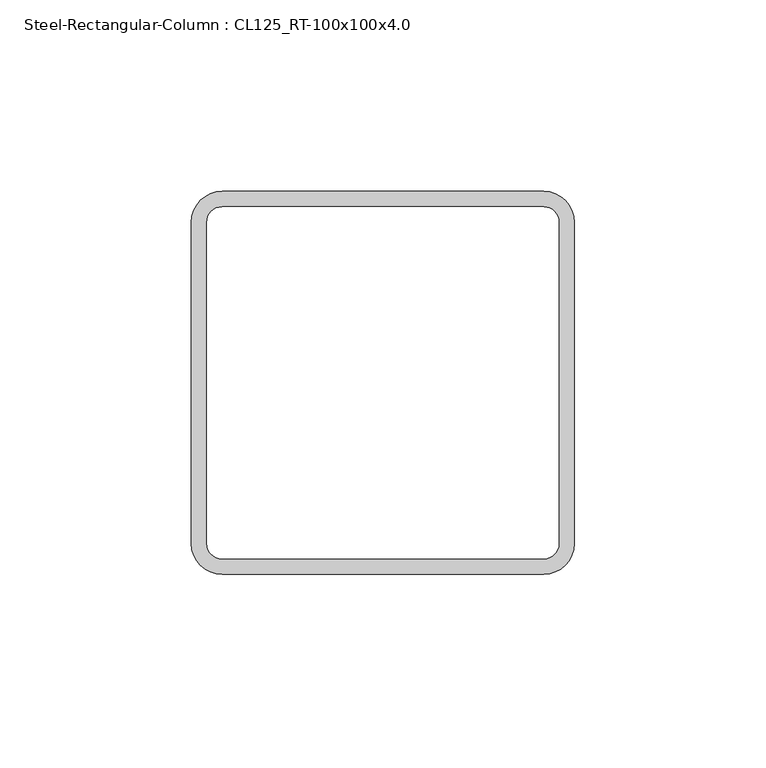
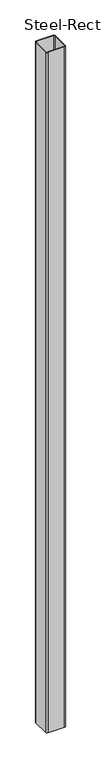
"""IFC4 building model written with IfcOpenShell, lengths in millimetres: column geometry, Steel-Rectangular-Column : CL125_RT-100x100x4.0."""

import ifcopenshell
import ifcopenshell.guid

model = None  # the IFC model being written
_history = None  # IfcOwnerHistory: only IFC2X3 demands one
_inside = {}  # id of a spatial element -> (the spatial element, [elements in it])
_under = {}  # id of a project, library or spatial element -> (it, [spatial elements below it])
_declared = {}  # id of a project -> (the project, [libraries it declares])
_typed = {}  # id of a type object -> (the type object, [elements of that type])
_made_of = {}  # id of a material, layer set ... -> (it, [elements and type objects made of it])


def new_model(schema):
    """Start an empty IFC model of exactly this schema.

    Asked for "IFC4X3", IfcOpenShell would pick the latest addendum, in which some entities
    have other attributes; the version numbers below select the first issue.
    IFC2X3 requires an IfcOwnerHistory on every rooted entity: one is made here for all.
    """
    global model, _history
    if schema == "IFC4X3":
        model = ifcopenshell.file(schema_version=(4, 3, 0, 0))
    else:
        model = ifcopenshell.file(schema=schema)
    _inside.clear()
    _under.clear()
    _declared.clear()
    _typed.clear()
    _made_of.clear()
    _history = None
    if model.schema == "IFC2X3":
        org = make("IfcOrganization", Name="unknown")
        user = make(
            "IfcPersonAndOrganization",
            ThePerson=make("IfcPerson", FamilyName="unknown"),
            TheOrganization=org,
        )
        app = make(
            "IfcApplication",
            ApplicationDeveloper=org,
            Version="unknown",
            ApplicationFullName="unknown",
            ApplicationIdentifier="unknown",
        )
        _history = make(
            "IfcOwnerHistory",
            OwningUser=user,
            OwningApplication=app,
            ChangeAction="ADDED",
            CreationDate=0,
        )
    return model


def make(cls, **values):
    """One entity of the class cls with the attributes given. An attribute that is None is left unset."""
    return model.create_entity(
        cls, **{name: value for name, value in values.items() if value is not None}
    )


def rooted(cls, **values):
    """An entity with a GlobalId (a new one), such as an element, a storey or a relation."""
    return make(cls, GlobalId=ifcopenshell.guid.new(), OwnerHistory=_history, **values)


def si_unit(unit_type, name, prefix=None):
    """IfcSIUnit, for example si_unit("LENGTHUNIT", "METRE", prefix="MILLI")."""
    return make("IfcSIUnit", UnitType=unit_type, Prefix=prefix, Name=name)


def assignment(units):
    """IfcUnitAssignment: the units of a project."""
    return None if units is None else make("IfcUnitAssignment", Units=units)


def point(xyz):
    """IfcCartesianPoint."""
    return None if xyz is None else make("IfcCartesianPoint", Coordinates=xyz)


def direction(xyz):
    """IfcDirection."""
    return None if xyz is None else make("IfcDirection", DirectionRatios=xyz)


def frame(location, z_axis=None, x_axis=None):
    """IfcAxis2Placement3D, a coordinate frame: its origin and axes. An axis left out is left unset."""
    return make(
        "IfcAxis2Placement3D",
        Location=point(location),
        Axis=direction(z_axis),
        RefDirection=direction(x_axis),
    )


def frame_2d(location, x_axis=None):
    """IfcAxis2Placement2D, a coordinate frame in the plane: its origin and x axis."""
    return make(
        "IfcAxis2Placement2D", Location=point(location), RefDirection=direction(x_axis)
    )


def origin():
    """The frame at (0, 0, 0) with its axes left unset."""
    return frame((0.0, 0.0, 0.0))


def place(relative_to, where):
    """IfcLocalPlacement: puts the frame where relative to a parent placement (None: the world)."""
    return make(
        "IfcLocalPlacement", PlacementRelTo=relative_to, RelativePlacement=where
    )


def context(
    kind, dimensions, precision=None, world=None, true_north=None, identifier=None
):
    """IfcGeometricRepresentationContext, for example the 3D "Model" context."""
    return make(
        "IfcGeometricRepresentationContext",
        ContextIdentifier=identifier,
        ContextType=kind,
        CoordinateSpaceDimension=dimensions,
        Precision=precision,
        WorldCoordinateSystem=world,
        TrueNorth=true_north,
    )


def project(units=None, contexts=None):
    """IfcProject with its units and contexts."""
    return rooted(
        "IfcProject",
        Name="project",
        RepresentationContexts=contexts,
        UnitsInContext=assignment(units),
    )


def spatial(cls, under=None, at=None, **own):
    """A site, building, storey or space (cls), placed at a placement, below another one or the project."""
    s = rooted(cls, ObjectPlacement=at, **own)
    if under is not None:
        _under.setdefault(under.id(), (under, []))[1].append(s)
    return s


def polyline(points):
    """IfcPolyline through the points."""
    return make("IfcPolyline", Points=[point(p) for p in points])


def circle_curve(where, radius):
    """IfcCircle in the frame where."""
    return make("IfcCircle", Position=where, Radius=radius)


def trimmed(basis, trim1, trim2, sense, master):
    """IfcTrimmedCurve: the piece of a basis curve between two trims."""
    return make(
        "IfcTrimmedCurve",
        BasisCurve=basis,
        Trim1=trim1,
        Trim2=trim2,
        SenseAgreement=sense,
        MasterRepresentation=master,
    )


def segment(curve, same_sense, transition):
    """IfcCompositeCurveSegment."""
    return make(
        "IfcCompositeCurveSegment",
        Transition=transition,
        SameSense=same_sense,
        ParentCurve=curve,
    )


def composite_curve(segments, self_intersect=None):
    """IfcCompositeCurve: segments joined end to end."""
    return make("IfcCompositeCurve", Segments=segments, SelfIntersect=self_intersect)


def outline(outer, holes=None, kind="AREA"):
    """IfcArbitraryClosedProfileDef: a profile drawn as a closed curve; with holes, ...WithVoids."""
    if holes is None:
        return make("IfcArbitraryClosedProfileDef", ProfileType=kind, OuterCurve=outer)
    return make(
        "IfcArbitraryProfileDefWithVoids",
        ProfileType=kind,
        OuterCurve=outer,
        InnerCurves=holes,
    )


def extrude(swept, where, along, depth):
    """IfcExtrudedAreaSolid: the profile swept, set in the frame where, extruded along a direction by depth."""
    return make(
        "IfcExtrudedAreaSolid",
        SweptArea=swept,
        Position=where,
        ExtrudedDirection=direction(along),
        Depth=depth,
    )


def shape(context_of_items, identifier, shape_type, items):
    """IfcShapeRepresentation: the items that make up one representation, for example the "Body"."""
    return make(
        "IfcShapeRepresentation",
        ContextOfItems=context_of_items,
        RepresentationIdentifier=identifier,
        RepresentationType=shape_type,
        Items=items,
    )


def source(mapping_origin, context_of_items, identifier, shape_type, items):
    """IfcRepresentationMap: a shape defined once, which mapped items show again and again."""
    return make(
        "IfcRepresentationMap",
        MappingOrigin=mapping_origin,
        MappedRepresentation=shape(context_of_items, identifier, shape_type, items),
    )


def transform(
    local_origin,
    x_axis=None,
    y_axis=None,
    z_axis=None,
    scale=None,
    scale2=None,
    scale3=None,
    uniform=True,
):
    """IfcCartesianTransformationOperator3D, or its non-uniform kind. x_axis, y_axis, z_axis: its Axis1, 2, 3."""
    if uniform:
        return make(
            "IfcCartesianTransformationOperator3D",
            Axis1=direction(x_axis),
            Axis2=direction(y_axis),
            LocalOrigin=point(local_origin),
            Scale=scale,
            Axis3=direction(z_axis),
        )
    return make(
        "IfcCartesianTransformationOperator3DnonUniform",
        Axis1=direction(x_axis),
        Axis2=direction(y_axis),
        LocalOrigin=point(local_origin),
        Scale=scale,
        Axis3=direction(z_axis),
        Scale2=scale2,
        Scale3=scale3,
    )


def mapped(mapping_source, mapping_target):
    """IfcMappedItem: shows the shape of a source again, moved by a transform."""
    return make(
        "IfcMappedItem", MappingSource=mapping_source, MappingTarget=mapping_target
    )


def made_of(thing, what):
    """Note that an element or type object is made of a material, layer set ...; save() writes the relation."""
    if what is not None:
        _made_of.setdefault(what.id(), (what, []))[1].append(thing)
    return thing


def element(
    cls,
    number,
    at=None,
    inside=None,
    cuts=None,
    type_object=None,
    material=None,
    context=None,
    identifier="Body",
    shape_type=None,
    held_by="IfcProductDefinitionShape",
    body=None,
    shapes=None,
    **own,
):
    """One element of the class cls, such as IfcWall. Its Tag is "e" and its number.

    at: its placement. inside: the storey or other place that contains it. cuts: it is an
    opening in that element (IfcRelVoidsElement). A single representation is given by context,
    identifier, shape_type and body (its items); several are given by shapes. held_by: the class
    of the entity that holds the representations. save() writes the other relations.
    """
    e = rooted(cls, Tag="e%d" % number, ObjectPlacement=at, **own)
    if body is not None:
        shapes = [shape(context, identifier, shape_type, body)]
    if shapes is not None:
        e.Representation = make(held_by, Representations=shapes)
    if inside is not None:
        _inside.setdefault(inside.id(), (inside, []))[1].append(e)
    if cuts is not None:
        rooted(
            "IfcRelVoidsElement", RelatingBuildingElement=cuts, RelatedOpeningElement=e
        )
    if type_object is not None:
        _typed.setdefault(type_object.id(), (type_object, []))[1].append(e)
    return made_of(e, material)


def aggregate(whole, parts):
    """IfcRelAggregates: a whole, such as a stair, and the parts it consists of."""
    return rooted("IfcRelAggregates", RelatingObject=whole, RelatedObjects=parts)


def save(model, path):
    """Write the relations noted so far, then the file.

    IfcRelAggregates (storeys below a building ...), IfcRelContainedInSpatialStructure (elements
    in a storey), IfcRelDefinesByType, IfcRelAssociatesMaterial and IfcRelDeclares: one each for
    every whole, place, type object, material and project.
    """
    for whole, parts in _under.values():
        aggregate(whole, parts)
    for where, things in _inside.values():
        rooted(
            "IfcRelContainedInSpatialStructure",
            RelatedElements=things,
            RelatingStructure=where,
        )
    for kind, things in _typed.values():
        rooted("IfcRelDefinesByType", RelatedObjects=things, RelatingType=kind)
    for what, things in _made_of.values():
        rooted("IfcRelAssociatesMaterial", RelatedObjects=things, RelatingMaterial=what)
    for by, libraries in _declared.values():
        rooted("IfcRelDeclares", RelatingContext=by, RelatedDefinitions=libraries)
    model.write(path)


def steel_rectangular_column_cl125_rt_100x100x4_0_3623087c(model_context):
    return source(origin(), model_context, "Body", "SweptSolid", [
        extrude(outline(composite_curve([segment(polyline([(42.0, -50.0), (-42.0, -50.0)]), True, "CONTINUOUS"), segment(trimmed(circle_curve(frame_2d((-42.0, -42.0)), 8.0), [point((-42.0, -50.0))], [point((-50.0, -42.0))], False, "CARTESIAN"), True, "CONTINUOUS"), segment(polyline([(-50.0, -42.0), (-50.0, 42.0)]), True, "CONTINUOUS"), segment(trimmed(circle_curve(frame_2d((-42.0, 42.0)), 8.0), [point((-50.0, 42.0))], [point((-42.0, 50.0))], False, "CARTESIAN"), True, "CONTINUOUS"), segment(polyline([(-42.0, 50.0), (42.0, 50.0)]), True, "CONTINUOUS"), segment(trimmed(circle_curve(frame_2d((42.0, 42.0)), 8.0), [point((42.0, 50.0))], [point((50.0, 42.0))], False, "CARTESIAN"), True, "CONTINUOUS"), segment(polyline([(50.0, 42.0), (50.0, -42.0)]), True, "CONTINUOUS"), segment(trimmed(circle_curve(frame_2d((42.0, -42.0)), 8.0), [point((50.0, -42.0))], [point((42.0, -50.0))], False, "CARTESIAN"), True, "CONTINUOUS")], self_intersect=False), holes=[composite_curve([segment(trimmed(circle_curve(frame_2d((42.0, -42.0)), 4.0), [point((42.0, -46.0))], [point((46.0, -42.0))], True, "CARTESIAN"), True, "CONTINUOUS"), segment(polyline([(46.0, -42.0), (46.0, 42.0)]), True, "CONTINUOUS"), segment(trimmed(circle_curve(frame_2d((42.0, 42.0)), 4.0), [point((46.0, 42.0))], [point((42.0, 46.0))], True, "CARTESIAN"), True, "CONTINUOUS"), segment(polyline([(42.0, 46.0), (-42.0, 46.0)]), True, "CONTINUOUS"), segment(trimmed(circle_curve(frame_2d((-42.0, 42.0)), 4.0), [point((-42.0, 46.0))], [point((-46.0, 42.0))], True, "CARTESIAN"), True, "CONTINUOUS"), segment(polyline([(-46.0, 42.0), (-46.0, -42.0)]), True, "CONTINUOUS"), segment(trimmed(circle_curve(frame_2d((-42.0, -42.0)), 4.0), [point((-46.0, -42.0))], [point((-42.0, -46.0))], True, "CARTESIAN"), True, "CONTINUOUS"), segment(polyline([(-42.0, -46.0), (42.0, -46.0)]), True, "CONTINUOUS")], self_intersect=False)]), frame((0.0, 0.0, 1400.0), z_axis=(0.0, 0.0, 1.0), x_axis=(1.0, 0.0, 0.0)), (0.0, 0.0, 1.0), 3600.0),
    ])


if __name__ == "__main__":
    model = new_model("IFC4")
    model_context = context("Model", 3, world=origin())
    ifc_project = project(units=[si_unit("LENGTHUNIT", "METRE", prefix="MILLI")], contexts=[model_context])
    site = spatial("IfcSite", under=ifc_project)
    building = spatial("IfcBuilding", under=site)
    placement = place(None, origin())
    steel_rectangular_column_cl125_rt_100x100x4_0_shape = steel_rectangular_column_cl125_rt_100x100x4_0_3623087c(model_context)
    element("IfcColumn", 1, ObjectType="Steel-Rectangular-Column : CL125_RT-100x100x4.0", at=placement, inside=building, context=model_context, shape_type="MappedRepresentation", body=[
        mapped(steel_rectangular_column_cl125_rt_100x100x4_0_shape, transform((0.0, 0.0, 0.0), x_axis=(1.0, 0.0, 0.0), y_axis=(0.0, 1.0, 0.0), z_axis=(0.0, 0.0, 1.0))),
    ])
    save(model, "model.ifc")

# Revit data of these elements
# Project information
#   Project ISM Data = "<?xml version=\"1.0\" encoding=\"utf-16\"?><ism schema_version=\"03.00\"><section_positioning><element family_name=\"CO_RC_REC\" symbol_name=\"CCC12_Rec_450x450\" section_id=\"F2ADF140-E21A-4820-8170-6F63D956DCAD\" category=\"OST_StructuralColumns\" mirror_y=\"0\" mirror_x=\"0\" /><element family_name=\"CO_RC_REC\" symbol_name=\"CCC12_Rec_450x450\" section_id=\"B35A310E-4F33-462b-819C-3ADD300C0CEB\" category=\"OST_StructuralColumns\" mirror_y=\"0\" mirror_x=\"0\" /><element family_name=\"CO_RC_REC\" symbol_name=\"CCC12_Rec_450x450\" section_id=\"711054EC-0DB2-46e3-AD20-004560300C00\" category=\"OST_StructuralColumns\" mirror_y=\"0\" mirror_x=\"0\" /><element family_name=\"CO_RC_REC\" symbol_name=\"300 x 450\" section_id=\"B5C54EC9-8EBD-4860-AB72-EF5791AED394\" category=\"OST_StructuralColumns\" mirror_y=\"0\" mirror_x=\"0\" /><element family_name=\"GI_RC_C\" symbol_name=\"SGC11_400x500\" section_id=\"0A7B8D02-9EA4-4aa9-A41A-E30BB5B6B6C5\" category=\"OST_StructuralFraming\" mirror_y=\"0\" mirror_x=\"0\" /><element family_name=\"GI_RC_C\" symbol_name=\"SGC11_400x500\" section_id=\"714BBD27-DB58-47da-B54C-5806291C2D3C\" category=\"OST_StructuralFraming\" mirror_y=\"0\" mirror_x=\"0\" /><element family_name=\"GI_RC_C\" symbol_name=\"SGC11_400x500\" section_id=\"F36E62C1-13EE-4807-A3C1-899E23E0BEDE\" category=\"OST_StructuralFraming\" mirror_y=\"0\" mirror_x=\"0\" /><element family_name=\"GI_RC_C\" symbol_name=\"SGC11_400x500\" section_id=\"F5448801-679E-44d6-8F46-E676344F8165\" category=\"OST_StructuralFraming\" mirror_y=\"0\" mirror_x=\"0\" /><element family_name=\"GI_RC_C\" symbol_name=\"SGC11_400x600\" section_id=\"05D74241-6318-4cac-95F5-7B878260D5B5\" category=\"OST_StructuralFraming\" mirror_y=\"0\" mirror_x=\"0\" /><element family_name=\"GI_RC_C\" symbol_name=\"SGC11_400x500\" section_id=\"846DCB0C-E06B-4978-9D43-E1CC0FDE7595\" category=\"OST_StructuralFraming\" mirror_y=\"0\" mirror_x=\"0\" /><element family_name=\"GI_RC_C\" symbol_name=\"SGC11_400x500\" section_id=\"2ADF82B8-986D-4f44-85DE-89D921292160\" category=\"OST_StructuralFraming\" mirror_y=\"0\" mirror_x=\"0\" /><element family_name=\"GI_RC_C\" symbol_name=\"SGC11_400x500\" section_id=\"7AF371ED-051B-4a30-8826-11F11C212B73\" category=\"OST_StructuralFraming\" mirror_y=\"0\" mirror_x=\"0\" /><element family_name=\"GI_RC_C\" symbol_name=\"SGC11_400x500\" section_id=\"2FE74006-ADDA-412f-A522-853919E62B4D\" category=\"OST_StructuralFraming\" mirror_y=\"0\" mirror_x=\"0\" /><element family_name=\"GI_RC_C\" symbol_name=\"SGC11_400x500\" section_id=\"09B63641-D581-4a6c-A18E-54C17EC989A4\" category=\"OST_StructuralFraming\" mirror_y=\"0\" mirror_x=\"0\" /><element family_name=\"GI_RC_C\" symbol_name=\"SGC11_400x500\" section_id=\"0DD6B52A-77D0-45a1-82B1-8236ED57078C\" category=\"OST_StructuralFraming\" mirror_y=\"0\" mirror_x=\"0\" /><element family_name=\"GI_RC_C\" symbol_name=\"SGC11_400x500\" section_id=\"35D311D2-DEB8-4469-97DE-110B6DF5B84D\" category=\"OST_StructuralFraming\" mirror_y=\"0\" mirror_x=\"0\" /><element family_name=\"GI_RC_C\" symbol_name=\"SGC11_400x500\" section_id=\"0D3CCDE5-CFF9-431b-A4BD-01BF6636D6BD\" category=\"OST_StructuralFraming\" mirror_y=\"0\" mirror_x=\"0\" /><element family_name=\"GI_RC_C\" symbol_name=\"SGC11_400x500\" section_id=\"C62B2A5B-024A-47ac-B030-C17A67E64A7B\" category=\"OST_StructuralFraming\" mirror_y=\"0\" mirror_x=\"0\" /><element family_name=\"GI_RC_C\" symbol_name=\"SGC11_400x500\" section_id=\"944C6E43-E607-48c3-8358-9E6CB88346E7\" category=\"OST_StructuralFraming\" mirror_y=\"0\" mirror_x=\"0\" /><element family_name=\"GI_RC_C\" symbol_name=\"SGC11_400x500\" section_id=\"A4B1F42D-B1C2-4ad2-8AD6-DB0D5E05998D\" category=\"OST_StructuralFraming\" mirror_y=\"0\" mirror_x=\"0\" /><element family_name=\"GI_RC_C\" symbol_name=\"SGC11_400x500\" section_id=\"007E6C70-1139-4b48-B003-C76FAD4C249A\" category=\"OST_StructuralFraming\" mirror_y=\"0\" mirror_x=\"0\" /><element family_name=\"GI_RC_C\" symbol_name=\"SGC11_400x500\" section_id=\"9941AC94-F03A-464c-9912-04590E0C31E0\" category=\"OST_StructuralFraming\" mirror_y=\"0\" mirror_x=\"0\" /><element family_name=\"GI_RC_C\" symbol_name=\"SGC11_400x500\" section_id=\"CFD98B8D-8FF4-4e71-A909-0FE7DBCE924E\" category=\"OST_StructuralFraming\" mirror_y=\"0\" mirror_x=\"0\" /><element family_name=\"GI_RC_C\" symbol_name=\"SGC11_400x500\" section_id=\"58262161-98E6-45c8-B2BD-4508105FF662\" category=\"OST_StructuralFraming\" mirror_y=\"0\" mirror_x=\"0\" /><element family_name=\"GI_RC_C\" symbol_name=\"SGC11_400x500\" section_id=\"66AB4841-610A-4883-97F7-1282A56484E1\" category=\"OST_StructuralFraming\" mirror_y=\"0\" mirror_x=\"0\" /><element family_name=\"GI_RC_C\" symbol_name=\"SGC11_400x500\" section_id=\"D2B324BE-BBD6-49da-9730-60EA7AD4D3A0\" category=\"OST_StructuralFraming\" mirror_y=\"0\" mirror_x=\"0\" /><element family_name=\"GI_RC_C\" symbol_name=\"SGC11_400x500\" section_id=\"92A8ECE7-C053-46b1-92ED-F2C041617E7B\" category=\"OST_StructuralFraming\" mirror_y=\"0\" mirror_x=\"0\" /><element family_name=\"GI_RC_C\" symbol_name=\"SGC11_400x500\" section_id=\"B4C4BDB0-65C4-4016-9C78-DBD77E229523\" category=\"OST_StructuralFraming\" mirror_y=\"0\" mirror_x=\"0\" /><element family_name=\"GI_RC_C\" symbol_name=\"SGC11_400x500\" section_id=\"57270646-162F-4c83-BDB7-A5FBEA9120BD\" category=\"OST_StructuralFraming\" mirror_y=\"0\" mirror_x=\"0\" /><element family_name=\"GI_RC_C\" symbol_name=\"SGC11_400x500\" section_id=\"BDEF733F-00AA-4eee-B6C6-50229FC1D236\" category=\"OST_StructuralFraming\" mirror_y=\"0\" mirror_x=\"0\" /><element family_name=\"GI_RC_C\" symbol_name=\"SGC11_400x500\" section_id=\"84A94E1E-3074-40f4-9690-97191755F019\" category=\"OST_StructuralFraming\" mirror_y=\"0\" mirror_x=\"0\" /><element family_name=\"GI_RC_C\" symbol_name=\"SGC11_400x500\" section_id=\"8A7D913D-7967-4718-912D-B83DF0AD2EDD\" category=\"OST_StructuralFraming\" mirror_y=\"0\" mirror_x=\"0\" /><element family_name=\"GI_RC_C\" symbol_name=\"SGC11_400x500\" section_id=\"83553D70-90FA-469c-B5C3-EF03F3FC6475\" category=\"OST_StructuralFraming\" mirror_y=\"0\" mirror_x=\"0\" /><element family_name=\"GI_RC_C\" symbol_name=\"SGC11_400x500\" section_id=\"6880C1E4-C50B-4c1b-B61C-23F2D8C46873\" category=\"OST_StructuralFraming\" mirror_y=\"0\" mirror_x=\"0\" /><element family_name=\"GI_RC_C\" symbol_name=\"SGC11_400x500\" section_id=\"08594C43-CD40-47de-A3BA-8BFB47F64994\" category=\"OST_StructuralFraming\" mirror_y=\"0\" mirror_x=\"0\" /><element family_name=\"GI_RC_C\" symbol_name=\"SGC11_400x500\" section_id=\"7D2E11FA-A5E1-4434-B9BE-AABA1A16CA03\" category=\"OST_StructuralFraming\" mirror_y=\"0\" mirror_x=\"0\" /><element family_name=\"GI_RC_C\" symbol_name=\"SGC11_400x500\" section_id=\"D892DFA4-5441-4ad2-A390-253492293B1B\" category=\"OST_StructuralFraming\" mirror_y=\"0\" mirror_x=\"0\" /><element family_name=\"GI_RC_C\" symbol_name=\"SGC11_400x500\" section_id=\"E5A32FE6-89C4-49f1-B3B9-1CABE7C48A4D\" category=\"OST_StructuralFraming\" mirror_y=\"0\" mirror_x=\"0\" /><element family_name=\"GI_RC_C\" symbol_name=\"SGC11_400x500\" section_id=\"8AE872C2-5DBE-47c5-934B-7E964A84B589\" category=\"OST_StructuralFraming\" mirror_y=\"0\" mirror_x=\"0\" /><element family_name=\"GI_RC_C\" symbol_name=\"SGC11_400x500\" section_id=\"3C847B60-488A-4604-A400-16A3A65E919B\" category=\"OST_StructuralFraming\" mirror_y=\"0\" mirror_x=\"0\" /><element family_name=\"GI_RC_C\" symbol_name=\"SGC11_400x500\" section_id=\"DBEC432A-3F7B-4266-AD99-2A937DC70BCF\" category=\"OST_StructuralFraming\" mirror_y=\"0\" mirror_x=\"0\" /><element family_name=\"GI_RC_C\" symbol_name=\"SGC11_400x500\" section_id=\"59403DD6-7A51-48aa-A3BE-962457E6F10E\" category=\"OST_StructuralFraming\" mirror_y=\"0\" mirror_x=\"0\" /><element family_name=\"GI_RC_C\" symbol_name=\"SGC11_400x500\" section_id=\"11CDDF5D-38B6-43b2-A291-FC188BE232BC\" category=\"OST_StructuralFraming\" mirror_y=\"0\" mirror_x=\"0\" /><element family_name=\"GI_RC_C\" symbol_name=\"SGC11_400x500\" section_id=\"10BF2843-EFC9-4136-933C-5B270D970277\" category=\"OST_StructuralFraming\" mirror_y=\"0\" mirror_x=\"0\" /><element family_name=\"GI_RC_C\" symbol_name=\"SGC11_400x500\" section_id=\"E1B09A9C-F6C6-47d9-976B-E313C0E3F52B\" category=\"OST_StructuralFraming\" mirror_y=\"0\" mirror_x=\"0\" /><element family_name=\"GI_RC_C\" symbol_name=\"SGC11_400x500\" section_id=\"A3A22EC3-26C8-4588-A0AB-AFAE02DF267E\" category=\"OST_StructuralFraming\" mirror_y=\"0\" mirror_x=\"0\" /><element family_name=\"GI_RC_C\" symbol_name=\"SGC11_400x500\" section_id=\"114828FC-BDC1-4343-9119-BCB5395DAA64\" category=\"OST_StructuralFraming\" mirror_y=\"0\" mirror_x=\"0\" /><element family_name=\"GI_RC_C\" symbol_name=\"SGC11_400x500\" section_id=\"797626F9-3558-4623-826F-15FB93088CB3\" category=\"OST_StructuralFraming\" mirror_y=\"0\" mirror_x=\"0\" /><element family_name=\"GI_RC_C\" symbol_name=\"SGC11_400x500\" section_id=\"4BF369CD-DF09-4346-96CB-C6C6380A2599\" category=\"OST_StructuralFraming\" mirror_y=\"0\" mirror_x=\"0\" /><element family_name=\"GI_RC_C\" symbol_name=\"SGC11_400x500\" section_id=\"722B46BA-61C4-44a1-9ECF-325B60B6688D\" category=\"OST_StructuralFraming\" mirror_y=\"0\" mirror_x=\"0\" /><element family_name=\"GI_RC_C\" symbol_name=\"SGC11_400x500\" section_id=\"C33DBE84-19C1-4379-AB6E-A41F7420F18C\" category=\"OST_StructuralFraming\" mirror_y=\"0\" mirror_x=\"0\" /><element family_name=\"GI_RC_C\" symbol_name=\"SGC11_400x500\" section_id=\"1F2D3B75-66F2-4d88-A1DD-647969477B86\" category=\"OST_StructuralFraming\" mirror_y=\"0\" mirror_x=\"0\" /><element family_name=\"GI_RC_C\" symbol_name=\"SGC11_400x500\" section_id=\"DFBF96B2-410A-4f39-80C4-D8CF78561C93\" category=\"OST_StructuralFraming\" mirror_y=\"0\" mirror_x=\"0\" /><element family_name=\"GI_RC_C\" symbol_name=\"SGC11_400x500\" section_id=\"D6793CD3-AB64-417c-9C28-8B18A0A2D336\" category=\"OST_StructuralFraming\" mirror_y=\"0\" mirror_x=\"0\" /><element family_name=\"GI_RC_C\" symbol_name=\"SGC11_400x500\" section_id=\"90884AC0-EA00-4caa-86E1-E6B886FD90ED\" category=\"OST_StructuralFraming\" mirror_y=\"0\" mirror_x=\"0\" /><element family_name=\"GI_RC_C\" symbol_name=\"SGC11_400x500\" section_id=\"64BC7B89-F7C8-4dae-A5C8-F10DF9E5F6BA\" category=\"OST_StructuralFraming\" mirror_y=\"0\" mirror_x=\"0\" /><element family_name=\"GI_RC_C\" symbol_name=\"SGC11_400x500\" section_id=\"D82E4D85-2728-40e5-9F60-1C7FB2990D78\" category=\"OST_StructuralFraming\" mirror_y=\"0\" mirror_x=\"0\" /><element family_name=\"GI_RC_C\" symbol_name=\"SGC11_400x500\" section_id=\"1E6D05B9-BF84-4669-AA27-948ADA1D511E\" category=\"OST_StructuralFraming\" mirror_y=\"0\" mirror_x=\"0\" /><element family_name=\"GI_RC_C\" symbol_name=\"SGC11_400x500\" section_id=\"73608CB2-EB94-466e-883D-814030EF49D6\" category=\"OST_StructuralFraming\" mirror_y=\"0\" mirror_x=\"0\" /><element family_name=\"GI_RC_C\" symbol_name=\"SGC11_400x500\" section_id=\"4EAF07EF-4E08-4065-9F08-BF69D4413867\" category=\"OST_StructuralFraming\" mirror_y=\"1\" mirror_x=\"1\" /></section_positioning><surface_member_mappings /><element_binding><element revit_id=\"0aa8b22b-49cd-4eb2-b994-d423f7aad482-0014435e\" ism_id=\"637A3C89-B4B9-4EE4-9E04-FF73E7A5771D\" /><element revit_id=\"af7cfdda-f71a-4a09-bb03-63e0c16d5d93-00152efa\" ism_id=\"088C1743-AFAE-4D55-B14F-2330F3A79060\" /><element revit_id=\"af7cfdda-f71a-4a09-bb03-63e0c16d5d93-00152efc\" ism_id=\"38278b30-864a-4bde-bfee-6c2d4309b281\" /><element revit_id=\"af7cfdda-f71a-4a09-bb03-63e0c16d5d93-00152eff\" ism_id=\"e2895b00-887b-4cf1-92a9-c4855f67b579\" /><element revit_id=\"af7cfdda-f71a-4a09-bb03-63e0c16d5d93-00152f02\" ism_id=\"a6b13b86-1938-47ee-8937-754844bb71d9\" /><element revit_id=\"af7cfdda-f71a-4a09-bb03-63e0c16d5d93-00152f05\" ism_id=\"b3cdb4ae-01be-49a8-8521-dfb37fcb7a09\" /><element revit_id=\"af7cfdda-f71a-4a09-bb03-63e0c16d5d93-00152f08\" ism_id=\"0a200294-2d0f-43b2-a10b-c345be42008c\" /><element revit_id=\"af7cfdda-f71a-4a09-bb03-63e0c16d5d
#     93-00152f0a\" ism_id=\"434ac00d-0b75-408a-b526-bf8655b26baf\" /><element revit_id=\"af7cfdda-f71a-4a09-bb03-63e0c16d5d93-00152f0c\" ism_id=\"5e4f7e2a-2154-47cc-93bc-24e7bd197632\" /><element revit_id=\"af7cfdda-f71a-4a09-bb03-63e0c16d5d93-00152f0e\" ism_id=\"f1998cd9-044c-4f7a-99e6-248bc5b45dba\" /><element revit_id=\"af7cfdda-f71a-4a09-bb03-63e0c16d5d93-00152f10\" ism_id=\"6ca0e144-6dd7-4824-b6a4-c3599ffcc64c\" /><element revit_id=\"af7cfdda-f71a-4a09-bb03-63e0c16d5d93-00152f12\" ism_id=\"173f1f07-ca52-4750-b7f6-1ef0180c36ba\" /><element revit_id=\"af7cfdda-f71a-4a09-bb03-63e0c16d5d93-00152f15\" ism_id=\"29a619d1-86ac-46c7-a220-2e78769b313e\" /><element revit_id=\"af7cfdda-f71a-4a09-bb03-63e0c16d5d93-00152f17\" ism_id=\"de21b25d-6b5e-4da6-89ee-8b671f1287ec\" /><element revit_id=\"af7cfdda-f71a-4a09-bb03-63e0c16d5d93-00152f19\" ism_id=\"70cdf538-eeaa-48c4-9315-181e56578638\" /><element revit_id=\"af7cfdda-f71a-4a09-bb03-63e0c16d5d93-00152f1b\" ism_id=\"49734cf8-a963-4163-b104-a25bff74fff0\" /><element revit_id=\"af7cfdda-f71a-4a09-bb03-63e0c16d5d93-00152f1d\" ism_id=\"a5a98e28-e98d-4759-bcab-d40632bfc19f\" /><element revit_id=\"af7cfdda-f71a-4a09-bb03-63e0c16d5d93-00152f1f\" ism_id=\"ab6af08f-90da-4d2f-a66a-db65621b8e94\" /><element revit_id=\"af7cfdda-f71a-4a09-bb03-63e0c16d5d93-00152f21\" ism_id=\"a65b64ab-134d-4223-82b7-5e66d90bc276\" /><element revit_id=\"af7cfdda-f71a-4a09-bb03-63e0c16d5d93-00152f23\" ism_id=\"6a1f317f-8940-4af8-9522-8e6c47c0c3a6\" /><element revit_id=\"af7cfdda-f71a-4a09-bb03-63e0c16d5d93-00152f25\" ism_id=\"880c6aab-7058-4382-9d83-6c759bdcf822\" /><element revit_id=\"af7cfdda-f71a-4a09-bb03-63e0c16d5d93-00152f27\" ism_id=\"555977b1-6494-4ee8-b235-8bae97762787\" /><element revit_id=\"af7cfdda-f71a-4a09-bb03-63e0c16d5d93-00152f29\" ism_id=\"66c9b467-8c65-4f1e-9542-95b43d793e9b\" /><element revit_id=\"af7cfdda-f71a-4a09-bb03-63e0c16d5d93-00152f2b\" ism_id=\"217a9ce2-64ab-4115-836e-06014fa1b21e\" /><element revit_id=\"af7cfdda-f71a-4a09-bb03-63e0c16d5d93-00152f2d\" ism_id=\"f7fc30da-832d-44e7-bab3-dd115d25639e\" /><element revit_id=\"af7cfdda-f71a-4a09-bb03-63e0c16d5d93-00152f2f\" ism_id=\"715eb46c-1b8d-4226-a7c6-6c6c165bf34d\" /><element revit_id=\"af7cfdda-f71a-4a09-bb03-63e0c16d5d93-00152f31\" ism_id=\"ef53c2b2-6fcf-42d2-96ea-f30a899bf64f\" /><element revit_id=\"af7cfdda-f71a-4a09-bb03-63e0c16d5d93-00152f34\" ism_id=\"1aefa093-18ee-4a97-8178-1b1fb4b7aceb\" /><element revit_id=\"af7cfdda-f71a-4a09-bb03-63e0c16d5d93-00152f38\" ism_id=\"262f02a9-64ca-487b-befd-4b58d44dffa7\" /><element revit_id=\"af7cfdda-f71a-4a09-bb03-63e0c16d5d93-00152f3b\" ism_id=\"6f2442a8-c4c0-4b53-9d7f-7059d6ededd2\" /><element revit_id=\"af7cfdda-f71a-4a09-bb03-63e0c16d5d93-00152f3e\" ism_id=\"dd838df4-69c7-406c-93e1-418c01f5734f\" /><element revit_id=\"af7cfdda-f71a-4a09-bb03-63e0c16d5d93-00152f40\" ism_id=\"9dec5077-28a7-4c32-95d2-08813de6a916\" /><element revit_id=\"af7cfdda-f71a-4a09-bb03-63e0c16d5d93-00152f42\" ism_id=\"9370ae5f-9277-4bb3-917b-cb3f318800a8\" /><element revit_id=\"af7cfdda-f71a-4a09-bb03-63e0c16d5d93-00152f44\" ism_id=\"0f3f2c81-58b4-4698-b1be-75061a4a2ae1\" /><element revit_id=\"af7cfdda-f71a-4a09-bb03-63e0c16d5d93-00152f46\" ism_id=\"95dca10f-6510-4ae7-a23e-7a1fd6939662\" /><element revit_id=\"af7cfdda-f71a-4a09-bb03-63e0c16d5d93-00152f49\" ism_id=\"83bad907-6a1c-4702-9990-a1a9c13d0160\" /><element revit_id=\"af7cfdda-f71a-4a09-bb03-63e0c16d5d93-00152f4d\" ism_id=\"7dba72dc-0de8-457c-8d3c-9c80941133ff\" /><element revit_id=\"af7cfdda-f71a-4a09-bb03-63e0c16d5d93-00152f51\" ism_id=\"a6cf3de2-949b-45b4-8029-061e06e5ab91\" /><element revit_id=\"af7cfdda-f71a-4a09-bb03-63e0c16d5d93-00152f54\" ism_id=\"77af5754-dd62-4c90-accb-d0b9405b5baf\" /><element revit_id=\"af7cfdda-f71a-4a09-bb03-63e0c16d5d93-00152f56\" ism_id=\"6461cb37-823d-49bb-bea2-3dbd4db85a81\" /><element revit_id=\"af7cfdda-f71a-4a09-bb03-63e0c16d5d93-00152f59\" ism_id=\"e2f2909f-27bc-426e-b2db-27b1217d3560\" /><element revit_id=\"af7cfdda-f71a-4a09-bb03-63e0c16d5d93-00152f5b\" ism_id=\"46c410de-fc65-4593-ae24-da1a154b45fb\" /><element revit_id=\"af7cfdda-f71a-4a09-bb03-63e0c16d5d93-00152f5d\" ism_id=\"d7d73cf7-a31f-421c-bc39-3ba338a334b1\" /><element revit_id=\"af7cfdda-f71a-4a09-bb03-63e0c16d5d93-00152f61\" ism_id=\"6bd81f7b-5fd8-4f19-ad3a-4e009274854c\" /><element revit_id=\"af7cfdda-f71a-4a09-bb03-63e0c16d5d93-00152f64\" ism_id=\"f25b9af0-504f-4aaf-a359-d2bc9d32b683\" /><element revit_id=\"af7cfdda-f71a-4a09-bb03-63e0c16d5d93-00152f66\" ism_id=\"f143dcd3-1cc7-47ae-b4ed-c960a7d1349c\" /><element revit_id=\"af7cfdda-f71a-4a09-bb03-63e0c16d5d93-00152f68\" ism_id=\"296e8d7f-a89b-405a-b793-fc1ea4b11be5\" /><element revit_id=\"af7cfdda-f71a-4a09-bb03-63e0c16d5d93-00152f6b\" ism_id=\"48b24488-3184-439c-b285-73e81edfef17\" /><element revit_id=\"af7cfdda-f71a-4a09-bb03-63e0c16d5d93-00152f6e\" ism_id=\"0db0ccd4-631c-4972-aad8-2fd483c55629\" /><element revit_id=\"af7cfdda-f71a-4a09-bb03-63e0c16d5d93-00152f71\" ism_id=\"ee51bd40-01d8-4a48-92c6-90509a96cad2\" /><element revit_id=\"af7cfdda-f71a-4a09-bb03-63e0c16d5d93-00152f73\" ism_id=\"e5c66ce6-ca9d-4591-9d75-5348307a88bc\" /><element revit_id=\"af7cfdda-f71a-4a09-bb03-63e0c16d5d93-00152f75\" ism_id=\"892d82ae-6f73-4af5-8575-78955f2b6c3b\" /><element revit_id=\"af7cfdda-f71a-4a09-bb03-63e0c16d5d93-00152f78\" ism_id=\"cb5b2a2e-5551-4b87-9d0b-6382c09e6ce2\" /><element revit_id=\"af7cfdda-f71a-4a09-bb03-63e0c16d5d93-00152f7c\" ism_id=\"1177c4ab-d04b-426b-80ba-afa1f1403e20\" /><element revit_id=\"af7cfdda-f71a-4a09-bb03-63e0c16d5d93-00152f7f\" ism_id=\"235d8a18-f10a-44ad-8945-ebb2f02646fa\" /><element revit_id=\"af7cfdda-f71a-4a09-bb03-63e0c16d5d93-00152f83\" ism_id=\"6127db9d-7d4b-44c8-806c-e4f7d278db0c\" /><element revit_id=\"af7cfdda-f71a-4a09-bb03-63e0c16d5d93-00152f86\" ism_id=\"85d79da8-d317-4e5b-88a2-88d20cb73d7d\" /><element revit_id=\"af7cfdda-f71a-4a09-bb03-63e0c16d5d93-00152f89\" ism_id=\"f4105a19-7c5e-4970-9446-50e578b67af2\" /><element revit_id=\"af7cfdda-f71a-4a09-bb03-63e0c16d5d93-00152f8b\" ism_id=\"ab299061-87b1-4edc-8a5c-c55542368f39\" /><element revit_id=\"af7cfdda-f71a-4a09-bb03-63e0c16d5d93-00152f8d\" ism_id=\"43097401-25be-48d4-a7ba-f3c37c1b84e9\" /><element revit_id=\"af7cfdda-f71a-4a09-bb03-63e0c16d5d93-00152f8f\" ism_id=\"fd9214b7-59e9-4736-b544-a37d4c180e24\" /><element revit_id=\"af7cfdda-f71a-4a09-bb03-63e0c16d5d93-00152f91\" ism_id=\"b83d1d95-2d97-4532-8a94-368577601c17\" /><element revit_id=\"af7cfdda-f71a-4a09-bb03-63e0c16d5d93-00152f94\" ism_id=\"9bd5e620-e2eb-4ede-9a8b-b0183e171248\" /><element revit_id=\"af7cfdda-f71a-4a09-bb03-63e0c16d5d93-00152f97\" ism_id=\"d6f9d903-1605-43dc-872c-2f9de6642af6\" /><element revit_id=\"af7cfdda-f71a-4a09-bb03-63e0c16d5d93-00152f99\" ism_id=\"7c236b12-3da8-4ae0-bc99-2aa089118476\" /><element revit_id=\"af7cfdda-f71a-4a09-bb03-63e0c16d5d93-00152f9b\" ism_id=\"2b88d03d-aeef-4f51-b98c-562513d6f6da\" /><element revit_id=\"af7cfdda-f71a-4a09-bb03-63e0c16d5d93-00152f9d\" ism_id=\"6639b07f-6759-4580-bc0a-91cdbc82216d\" /><element revit_id=\"af7cfdda-f71a-4a09-bb03-63e0c16d5d93-00152f9f\" ism_id=\"d17e7cf5-d760-4c38-8bb0-8a57fe45e3ad\" /><element revit_id=\"af7cfdda-f71a-4a09-bb03-63e0c16d5d93-00152fa2\" ism_id=\"6dbdf2a2-22ac-4132-a9ae-8992fe15b0d7\" /><element revit_id=\"af7cfdda-f71a-4a09-bb03-63e0c16d5d93-00152fa4\" ism_id=\"663381be-9f3f-499f-b7c1-64170401ecb3\" /><element revit_id=\"af7cfdda-f71a-4a09-bb03-63e0c16d5d93-00152fa6\" ism_id=\"5ba3ff14-3d24-47a8-9418-aecce16bd943\" /><element revit_id=\"af7cfdda-f71a-4a09-bb03-63e0c16d5d93-00152fa8\" ism_id=\"8f845e6a-1432-4c61-8362-e12c105320fb\" /><element revit_id=\"af7cfdda-f71a-4a09-bb03-63e0c16d5d93-00152faa\" ism_id=\"263897bf-02c2-4ed7-8e3f-2020d545125e\" /><element revit_id=\"af7cfdda-f71a-4a09-bb03-63e0c16d5d93-00152fac\" ism_id=\"f1241312-d990-4c87-92ff-afc1975a3d67\" /><element revit_id=\"af7cfdda-f71a-4a09-bb03-63e0c16d5d93-00152fae\" ism_id=\"5740cb23-0cbc-47ce-acea-31b5a043bf0c\" /><element revit_id=\"af7cfdda-f71a-4a09-bb03-63e0c16d5d93-00152fb0\" ism_id=\"7aeaeafb-f9bc-4bee-b237-caade22069b8\" /><element revit_id=\"af7cfdda-f71a-4a09-bb03-63e0c16d5d93-00152fb3\" ism_id=\"90084dda-e197-4e46-8e5b-4f629a594830\" /><element revit_id=\"af7cfdda-f71a-4a09-bb03-63e0c16d5d93-00152fb5\" ism_id=\"2c392f12-2b50-4bd2-8c41-ef64640e587b\" /><element revit_id=\"af7cfdda-f71a-4a09-bb03-63e0c16d5d93-00152fb7\" ism_id=\"d25284c0-6931-4cbb-8ed3-63397f6a5616\" /><element revit_id=\"af7cfdda-f71a-4a09-bb03-63e0c16d5d93-00152fb9\" ism_id=\"32799d39-e9bc-468c-ac64-a3f2c8e075af\" /><element revit_id=\"af7cfdda-f71a-4a09-bb03-63e0c16d5d93-00152fbb\" ism_id=\"61a092b8-d924-4e61-a1ef-adc051541aaf\" /><element revit_id=\"af7cfdda-f71a-4a09-bb03-63e0c16d5d93-00152fbe\" ism_id=\"ae89ad42-0006-42ee-9328-01a896002b7a\" /><element revit_id=\"af7cfdda-f71a-4a09-bb03-63e0c16d5d93-00152fc0\" ism_id=\"7b4d47fd-5fcd-4692-9b39-36bb95372647\" /><element revit_id=\"af7cfdda-f71a-4a09-bb03-63e0c16d5d93-00152fc2\" ism_id=\"150f022d-eb78-47d8-8d70-c7ea5433f366\" /><element revit_id=\"af7cfdda-f71a-4a09-bb03-63e0c16d5d93-00152fc4\" ism_id=\"6780451e-52c6-4962-8bb4-f1fd57bf7865\" /><element revit_id=\"af7cfdda-f71a-4a09-bb03-63e0c16d5d93-00152fc6\" ism_id=\"b3896748-2d7c-424b-ae81-8b769d840fbc\" /><element revit_id=\"af7cfdda-f71a-4a09-bb03-63e0c16d5d93-00152fc9\" ism_id=\"0c64c745-ce95-4f37-8a9d-d07fd5d17ecb\" /><element revit_id=\"af7cfdda-f71a-4a09-bb03-63e0c16d5d93-00152fcc\" ism_id=\"dc23390d-d501-4d7e-9369-f7793a7306a7\" /><element revit_id=\"af7cfdda-f71a-4a09-bb03-63e0c16d5d93-00152fcf\" ism_id=\"a2d2dfc7-08e7-459b-9de9-2d46c1b9d65d\" /><element revit_id=\"af7cfdda-f71a-4a09-bb03-63e0c16d5d93-00152fd2\" ism_id=\"0357c393-c221-46b8-a525-7eece05024d5\" /><element revit_id=\"af7cfdda-f71a-4a09-bb03-63e0c16d5d93-00152fd4\" ism_id=\"7514ec1a-cc54-428f-bbfe-53465c7b9971\" /><element revit_id=\"af7cfdda-f71a-4a09-bb03-63e0c16d5d93-00152fd7\" ism_id=\"f5e61f1a-565d-4eed-b8cc-74798bf49f83\" /><element revit_id=\"af7cfdda-f71a-4a09-bb03-63e0c16d5d93-00152fd9\" ism_id=\"7d7031a0-6061-49e6-8bb3-df1503ddb602\" /><element revit_id=\"af7cfdda-f71a-4a09-bb03-63e0c16d5d93-00152fdb\" ism_id=\"0d733cbc-e2dd-44ec-a5f3-da43d2d7ec46\" /><element revit_id=\"af7cfdda-f71a-4a09-bb03-63e0c16d5d93-00152fdd\" ism_id=\"21cbc8e9-c640-4a2e-8958-1d3b7a784879\" /><element revit_id=\"af7cfdda-f71a-4a09-bb03-63e0c16d5d93-00152fdf\" ism_id=\"fac86bbb-1d81-4320-81cd-30997be31eb4\" /><element revit_id=\"af7cfdda-f71a-4a09-bb03-63e0c16d5d93-00152fe1\" ism_id=\"ebc7c696-170e-4ba4-8599-103279d331b8\" /><element revit_id=\"af7cfdda-f71a-4a09-bb03-63e0c16d5d93-00152fe3\" ism_id=\"91dec439-7fd8-4259-bbce-df46237765e2\" /><element revit_id=\"af7cfdda-f71a-4a09-bb03-63e0c16d5d93-00152fe5\" ism_id=\"6227503a-c521-4b5a-b5c3-b9e2ea2b5c81\" /><element revit_id=\"af7cfdda-f71a-4a09-bb03-63e0c16d5d93-00152fe7\" ism_id=\"e6e91966-53ab-4536-84a0-3f6e5a22fbeb\" /><element revit_id=\"af7cfdda-f71a-4a09-bb03-63e0c16d5d93-00152fe9\" ism_id=\"fb3387b3-301c-40a5-8217-97be67c50843\" /><element revit_id=\"af7cfdda-f71a-4a09-bb03-63e0c16d5d93-00152feb\" ism_id=\"37825fc8-0fe2-440e-933a-1453c922c9d9\" /><element revit_id=\"af7cfdda-f71a-4a09-bb03-63e0c16d5d93-00152fed\" ism_id=\"06b175df-5526-4920-a3d6-7f2ff872756e\" /><element revit_id=\"af7cfdda-f71a-4a09-bb03-63e0c16d5d93-00152fef\" ism_id=\"a8fbce7a-6989-46e5-9bc5-c497d4a295c9\" /><element revit_id=\"af7cfdda-f71a-4a09-bb03-63e0c16d5d93-00152ff1\" ism_id=\"cf8ccf89-d0da-4b4e-93d8-85d639853d5e\" /><element revit_id=\"af7cfdda-f71a-4a09-bb03-63e0c16d5d93-00152ff3\" ism_id=\"1b85e87c-6c2a-4057-8491-40e4237cd0e6\" /><element revit_id=\"af7cfdda-f71a-4a09-bb03-63e0c16d5d93-00152ff5\" ism_id=\"69be497f-343c-4d38-9ea0-e959474332f8\" /><element revit_id=\"af7cfdda-f71a-4a09-bb03-63e0c16d5d93-00152ff7\" ism_id=\"72738956-f87a-41b4-a019-35adc3bff764\" /><element revit_id=\"af7cfdda-f71a-4a09-bb03-63e0c16d5d93-00152ff9\" ism_id=\"f127b15c-142d-4b57-83a6-5b76ac4cde6e\" /><element revit_id=
#     \"af7cfdda-f71a-4a09-bb03-63e0c16d5d93-00152ffb\" ism_id=\"3a38a709-bfa8-404e-b889-5af5e78ea0bf\" /><element revit_id=\"af7cfdda-f71a-4a09-bb03-63e0c16d5d93-00152ffe\" ism_id=\"bebf0363-7e59-4a43-8f5b-502fcc4a338d\" /><element revit_id=\"af7cfdda-f71a-4a09-bb03-63e0c16d5d93-00153000\" ism_id=\"157fe154-0d28-4e8c-a143-e2896867fd28\" /><element revit_id=\"af7cfdda-f71a-4a09-bb03-63e0c16d5d93-00153002\" ism_id=\"1bf52bf8-7327-4d55-b5cd-bf7c9bf89688\" /><element revit_id=\"af7cfdda-f71a-4a09-bb03-63e0c16d5d93-00153005\" ism_id=\"7a0025bf-d54b-4614-9002-7bd4a82da90e\" /><element revit_id=\"af7cfdda-f71a-4a09-bb03-63e0c16d5d93-00153008\" ism_id=\"cad53638-8c8f-4a89-ab6f-d8a32131833b\" /><element revit_id=\"af7cfdda-f71a-4a09-bb03-63e0c16d5d93-0015300a\" ism_id=\"05672ccd-1a96-434c-8da1-7a706b3561f7\" /><element revit_id=\"af7cfdda-f71a-4a09-bb03-63e0c16d5d93-0015300c\" ism_id=\"bb809016-b2bb-4157-847e-1cca3692ba19\" /><element revit_id=\"af7cfdda-f71a-4a09-bb03-63e0c16d5d93-0015300f\" ism_id=\"720ed192-8aa7-46fd-9f7a-15d64351767c\" /><element revit_id=\"af7cfdda-f71a-4a09-bb03-63e0c16d5d93-00153011\" ism_id=\"9a47cdb9-976d-41f3-a5c3-5a7516a7763c\" /><element revit_id=\"af7cfdda-f71a-4a09-bb03-63e0c16d5d93-00153013\" ism_id=\"aba01787-c82b-453e-8db2-70277a34d5ad\" /><element revit_id=\"af7cfdda-f71a-4a09-bb03-63e0c16d5d93-00153015\" ism_id=\"f6b882e3-d64a-44b1-878c-9c00ee1fde86\" /><element revit_id=\"af7cfdda-f71a-4a09-bb03-63e0c16d5d93-00153017\" ism_id=\"95108815-490a-427a-aec1-8fcefc57c858\" /><element revit_id=\"af7cfdda-f71a-4a09-bb03-63e0c16d5d93-00153019\" ism_id=\"8fe55cf1-56b4-4a62-948a-d7f0c95bd04b\" /><element revit_id=\"af7cfdda-f71a-4a09-bb03-63e0c16d5d93-0015301b\" ism_id=\"b889bf8b-3bdd-410a-b11b-9ca69449d470\" /><element revit_id=\"af7cfdda-f71a-4a09-bb03-63e0c16d5d93-0015301d\" ism_id=\"ef8604de-de5b-45ec-9158-0b702e6ef713\" /><element revit_id=\"af7cfdda-f71a-4a09-bb03-63e0c16d5d93-0015301f\" ism_id=\"40ee286a-4bc9-4d4f-ba6d-fe1ac9da03cf\" /><element revit_id=\"af7cfdda-f71a-4a09-bb03-63e0c16d5d93-00153021\" ism_id=\"cc903f39-6bdf-4081-a56c-883169221735\" /><element revit_id=\"af7cfdda-f71a-4a09-bb03-63e0c16d5d93-00153023\" ism_id=\"0af04955-dcb6-4295-b3d4-7c432a233062\" /><element revit_id=\"af7cfdda-f71a-4a09-bb03-63e0c16d5d93-00153025\" ism_id=\"75a51549-6a04-4399-b818-f170a8c10286\" /><element revit_id=\"af7cfdda-f71a-4a09-bb03-63e0c16d5d93-00153027\" ism_id=\"7e183794-5c66-46bc-97f5-2df209b3286d\" /><element revit_id=\"af7cfdda-f71a-4a09-bb03-63e0c16d5d93-00153029\" ism_id=\"ed4a7448-29b0-44e3-8b6f-7310f83440ab\" /><element revit_id=\"af7cfdda-f71a-4a09-bb03-63e0c16d5d93-0015302b\" ism_id=\"fdb5eb17-b94e-40c1-b703-3ecb5e4efee4\" /><element revit_id=\"af7cfdda-f71a-4a09-bb03-63e0c16d5d93-0015302d\" ism_id=\"779397c1-65b7-447f-a72e-2a09308021ea\" /><element revit_id=\"af7cfdda-f71a-4a09-bb03-63e0c16d5d93-0015302f\" ism_id=\"7b409707-86c5-44e2-919e-92ad5bb9eb8b\" /><element revit_id=\"af7cfdda-f71a-4a09-bb03-63e0c16d5d93-00153031\" ism_id=\"d337c78b-590d-406c-bf20-6a3558821db1\" /><element revit_id=\"af7cfdda-f71a-4a09-bb03-63e0c16d5d93-00153033\" ism_id=\"c27f5f6d-8445-4415-853d-d316787bea6e\" /><element revit_id=\"af7cfdda-f71a-4a09-bb03-63e0c16d5d93-00153035\" ism_id=\"76036a55-3bab-417a-ba41-ec1335e2e2a7\" /><element revit_id=\"af7cfdda-f71a-4a09-bb03-63e0c16d5d93-00153037\" ism_id=\"24be638c-ff89-4616-8974-5b79c81e6e56\" /><element revit_id=\"af7cfdda-f71a-4a09-bb03-63e0c16d5d93-00153039\" ism_id=\"015f9f2c-2353-4795-b891-e4ee986f25f7\" /><element revit_id=\"af7cfdda-f71a-4a09-bb03-63e0c16d5d93-0015303b\" ism_id=\"91f8ddfb-c5b9-4f33-b141-a6edfbccf098\" /><element revit_id=\"af7cfdda-f71a-4a09-bb03-63e0c16d5d93-0015303d\" ism_id=\"78540364-1ba5-4f0c-95fb-ba8631e32695\" /><element revit_id=\"af7cfdda-f71a-4a09-bb03-63e0c16d5d93-0015303f\" ism_id=\"9d53e406-367b-4e3e-b5e8-d421731e1aab\" /><element revit_id=\"af7cfdda-f71a-4a09-bb03-63e0c16d5d93-00153041\" ism_id=\"24aa6051-1a20-4f08-8962-6f6f9ff4dc98\" /><element revit_id=\"af7cfdda-f71a-4a09-bb03-63e0c16d5d93-00153043\" ism_id=\"572a4144-5250-4962-a1b9-09502cda2774\" /><element revit_id=\"af7cfdda-f71a-4a09-bb03-63e0c16d5d93-00153045\" ism_id=\"1f486980-0be9-4aad-b32e-0608218bf68e\" /><element revit_id=\"af7cfdda-f71a-4a09-bb03-63e0c16d5d93-00153047\" ism_id=\"588ed856-d113-4521-b97c-a4d7ac7ba406\" /><element revit_id=\"af7cfdda-f71a-4a09-bb03-63e0c16d5d93-00153049\" ism_id=\"741942b7-995d-48cb-8401-4faec8ef8d15\" /><element revit_id=\"af7cfdda-f71a-4a09-bb03-63e0c16d5d93-0015304b\" ism_id=\"85254c30-08c9-46e3-acd6-6b5131f485ce\" /><element revit_id=\"af7cfdda-f71a-4a09-bb03-63e0c16d5d93-0015304e\" ism_id=\"2d57d6c0-67d8-48bd-b16f-8ef7edb485b1\" /><element revit_id=\"af7cfdda-f71a-4a09-bb03-63e0c16d5d93-00153050\" ism_id=\"57b4caff-473e-4ebc-b42c-d73ce4ca67d8\" /><element revit_id=\"af7cfdda-f71a-4a09-bb03-63e0c16d5d93-00153052\" ism_id=\"1adae240-a487-478c-a898-61bee40e7415\" /><element revit_id=\"af7cfdda-f71a-4a09-bb03-63e0c16d5d93-00153054\" ism_id=\"62613b5f-092e-4f63-86ac-d3e070a85bc5\" /><element revit_id=\"af7cfdda-f71a-4a09-bb03-63e0c16d5d93-00153056\" ism_id=\"6aecb1de-b991-4eed-80ad-e1b9ccc03a87\" /><element revit_id=\"af7cfdda-f71a-4a09-bb03-63e0c16d5d93-00153058\" ism_id=\"ecab5d8d-84d0-44a4-9549-bca959ac514b\" /><element revit_id=\"af7cfdda-f71a-4a09-bb03-63e0c16d5d93-0015305a\" ism_id=\"589f44ad-061b-46bc-91bd-bf9b1e708415\" /><element revit_id=\"af7cfdda-f71a-4a09-bb03-63e0c16d5d93-0015305c\" ism_id=\"bfa24af8-499f-45ff-9e9d-d5cc0761fed6\" /><element revit_id=\"af7cfdda-f71a-4a09-bb03-63e0c16d5d93-0015305e\" ism_id=\"8114f473-ca73-4cc8-b3e2-979f07368f66\" /><element revit_id=\"af7cfdda-f71a-4a09-bb03-63e0c16d5d93-00153060\" ism_id=\"4dde7439-2ac9-412f-a5f5-e9fd0f294ec8\" /><element revit_id=\"af7cfdda-f71a-4a09-bb03-63e0c16d5d93-00153062\" ism_id=\"661cc7d8-fd9c-4505-b43e-241bfd24b2d0\" /><element revit_id=\"af7cfdda-f71a-4a09-bb03-63e0c16d5d93-00153064\" ism_id=\"1e7f186f-1b55-4d4c-bf9f-18595049605e\" /><element revit_id=\"af7cfdda-f71a-4a09-bb03-63e0c16d5d93-00153066\" ism_id=\"ee968183-c9c6-4eab-86cf-0eda12de724b\" /><element revit_id=\"af7cfdda-f71a-4a09-bb03-63e0c16d5d93-00153068\" ism_id=\"5de1f319-cdd1-4b9a-8f8e-b86394effa22\" /><element revit_id=\"af7cfdda-f71a-4a09-bb03-63e0c16d5d93-0015306a\" ism_id=\"fa557a6c-2e39-4481-9eb5-5ede8fd31c49\" /><element revit_id=\"af7cfdda-f71a-4a09-bb03-63e0c16d5d93-0015306c\" ism_id=\"b2710e8e-0f5f-4e74-a366-aef04da22cd3\" /><element revit_id=\"af7cfdda-f71a-4a09-bb03-63e0c16d5d93-0015306e\" ism_id=\"5633c3b7-f903-46ee-b126-8a20a9a62c90\" /><element revit_id=\"af7cfdda-f71a-4a09-bb03-63e0c16d5d93-00153070\" ism_id=\"62796ef8-c4bb-4b9f-bd14-cc7392046eb4\" /><element revit_id=\"af7cfdda-f71a-4a09-bb03-63e0c16d5d93-00153072\" ism_id=\"db898ada-150e-4ff5-a9f8-16e27b46b754\" /><element revit_id=\"af7cfdda-f71a-4a09-bb03-63e0c16d5d93-00153075\" ism_id=\"d3965d2d-e119-4f6b-af8d-52c8a5397d36\" /><element revit_id=\"af7cfdda-f71a-4a09-bb03-63e0c16d5d93-00153077\" ism_id=\"063574e4-6319-4ba7-8e34-1638a1357d5f\" /><element revit_id=\"af7cfdda-f71a-4a09-bb03-63e0c16d5d93-00153079\" ism_id=\"6de69805-8980-44f0-9316-6d50d1b47cbb\" /><element revit_id=\"af7cfdda-f71a-4a09-bb03-63e0c16d5d93-0015307b\" ism_id=\"e5f77c5b-4806-4993-8875-6149db708e42\" /><element revit_id=\"af7cfdda-f71a-4a09-bb03-63e0c16d5d93-0015307d\" ism_id=\"a13071c9-c086-4896-95a6-a015bc531f25\" /><element revit_id=\"af7cfdda-f71a-4a09-bb03-63e0c16d5d93-0015307f\" ism_id=\"c9d216f9-adca-4752-b8c1-d779727505dd\" /><element revit_id=\"af7cfdda-f71a-4a09-bb03-63e0c16d5d93-00153081\" ism_id=\"5b167621-3850-4169-8bee-1e0420bf6050\" /><element revit_id=\"af7cfdda-f71a-4a09-bb03-63e0c16d5d93-00153083\" ism_id=\"09cf76ae-a083-4203-a622-7e9424374f66\" /><element revit_id=\"af7cfdda-f71a-4a09-bb03-63e0c16d5d93-00153085\" ism_id=\"14063b50-058d-464a-aa08-369865983eeb\" /><element revit_id=\"af7cfdda-f71a-4a09-bb03-63e0c16d5d93-00153087\" ism_id=\"add5837f-63be-4349-b708-9f4051059e25\" /><element revit_id=\"af7cfdda-f71a-4a09-bb03-63e0c16d5d93-00153089\" ism_id=\"b4c60bd3-61cb-423f-916a-fa2b71585228\" /><element revit_id=\"af7cfdda-f71a-4a09-bb03-63e0c16d5d93-0015308b\" ism_id=\"6251d90e-381f-4771-818c-f7465ae91864\" /><element revit_id=\"af7cfdda-f71a-4a09-bb03-63e0c16d5d93-0015308d\" ism_id=\"7693be9d-48ca-4005-bed4-90e9c08d3a38\" /><element revit_id=\"af7cfdda-f71a-4a09-bb03-63e0c16d5d93-0015308f\" ism_id=\"a6a39ca9-cd56-43ba-bfe8-2cf3b78878cc\" /><element revit_id=\"af7cfdda-f71a-4a09-bb03-63e0c16d5d93-00153091\" ism_id=\"1a3956c4-77bb-4ccc-a12d-c3514cf365d4\" /><element revit_id=\"af7cfdda-f71a-4a09-bb03-63e0c16d5d93-00153093\" ism_id=\"2ffa7a89-8ee9-470a-b3d8-7c27f566e226\" /><element revit_id=\"af7cfdda-f71a-4a09-bb03-63e0c16d5d93-00153095\" ism_id=\"e865b460-944f-4057-a6e8-4e39cb88d97d\" /><element revit_id=\"af7cfdda-f71a-4a09-bb03-63e0c16d5d93-00153097\" ism_id=\"69410bb9-8440-4a88-9151-b5459095fe2e\" /><element revit_id=\"af7cfdda-f71a-4a09-bb03-63e0c16d5d93-00153099\" ism_id=\"1efae87b-0246-432c-a428-82c87fb3929c\" /><element revit_id=\"af7cfdda-f71a-4a09-bb03-63e0c16d5d93-0015309b\" ism_id=\"e1d5fb57-3b5d-4a32-bccb-cea278671f2f\" /><element revit_id=\"af7cfdda-f71a-4a09-bb03-63e0c16d5d93-0015309d\" ism_id=\"c74a7061-f4b2-41b5-b3ff-caf6cf9dfffd\" /><element revit_id=\"af7cfdda-f71a-4a09-bb03-63e0c16d5d93-0015309f\" ism_id=\"aa777ec3-1257-49eb-b597-fbab7bda8b11\" /><element revit_id=\"af7cfdda-f71a-4a09-bb03-63e0c16d5d93-001530a1\" ism_id=\"7420a67b-bb48-477d-823a-c473ce92c083\" /><element revit_id=\"af7cfdda-f71a-4a09-bb03-63e0c16d5d93-001530a3\" ism_id=\"1ee9340a-8778-4cd6-be2d-57fb5fe16e45\" /><element revit_id=\"af7cfdda-f71a-4a09-bb03-63e0c16d5d93-001530a5\" ism_id=\"3216ac21-29b0-45a7-a070-99a114df4980\" /><element revit_id=\"af7cfdda-f71a-4a09-bb03-63e0c16d5d93-001530a7\" ism_id=\"dce9c5c3-a57a-4091-8398-cace2e63f290\" /><element revit_id=\"af7cfdda-f71a-4a09-bb03-63e0c16d5d93-001530a9\" ism_id=\"dcadcd2e-1b12-41e7-a9d5-5d99303c7e51\" /><element revit_id=\"af7cfdda-f71a-4a09-bb03-63e0c16d5d93-001530ab\" ism_id=\"ed4bf433-a5ea-40d4-8551-b735160eed03\" /><element revit_id=\"af7cfdda-f71a-4a09-bb03-63e0c16d5d93-001530ad\" ism_id=\"2cd91197-39b9-4301-8775-b1530f8812f8\" /><element revit_id=\"af7cfdda-f71a-4a09-bb03-63e0c16d5d93-001530af\" ism_id=\"53460b48-5382-4fff-98f2-ab500700bbca\" /><element revit_id=\"af7cfdda-f71a-4a09-bb03-63e0c16d5d93-001530b1\" ism_id=\"0d733cb9-b11e-45a1-89e1-53989b2ba4d5\" /><element revit_id=\"af7cfdda-f71a-4a09-bb03-63e0c16d5d93-001530b3\" ism_id=\"9b6990cb-bf48-452d-9572-952a8acd923b\" /><element revit_id=\"af7cfdda-f71a-4a09-bb03-63e0c16d5d93-001530b5\" ism_id=\"edb53df5-f0f8-45af-a38d-8c910b94c4aa\" /><element revit_id=\"af7cfdda-f71a-4a09-bb03-63e0c16d5d93-001530b7\" ism_id=\"a42a99cd-d791-460b-b7db-769eef45d4ee\" /><element revit_id=\"af7cfdda-f71a-4a09-bb03-63e0c16d5d93-001530b9\" ism_id=\"473eafff-0971-4b1a-8b61-a7662a5d0782\" /><element revit_id=\"af7cfdda-f71a-4a09-bb03-63e0c16d5d93-001530bb\" ism_id=\"b801d819-54a6-4fd3-91e7-5d49978bee50\" /><element revit_id=\"af7cfdda-f71a-4a09-bb03-63e0c16d5d93-001530bd\" ism_id=\"aa72d39c-13a9-4733-9528-98e90ae2a493\" /><element revit_id=\"af7cfdda-f71a-4a09-bb03-63e0c16d5d93-001530c0\" ism_id=\"e50950ab-c982-40e9-a130-a8fe9c5071aa\" /><element revit_id=\"af7cfdda-f71a-4a09-bb03-63e0c16d5d93-001530c3\" ism_id=\"caa8c896-9dda-4bb9-b942-fab7d7988525\" /><element revit_id=\"af7cfdda-f71a-4a09-bb03-63e0c16d5d93-001530c5\" ism_id=\"45f4fe9a-436c-4b4d-a48d-573edf59a390\" /><element revit_id=\"af7cfdda-f71a-4a09-bb03-63e0c16d5d93-001530c7\" ism_id=\"eb513efb-1058-4d3f-8f19-56219176a71a\" /><element revit_id=\"af7cfdda-f71a-4a09-bb03-63e0c16d5d93-001530c9\" ism_id=\"537abf12-3423-4f70-8613-a81d434152a6\" /><element revit_id=\"af7cfdda-f71a-4a09-bb03-63e0c16d5d93-001530cb\" ism_id=\"683f9f6d-960e-4ae9-ad7f-39eee39c3d47\" /><element revit_id=\"af7cfdda-f71a-4a09-bb03-63e0c16d5d93-001530cd\" ism_id=\"2ceed54c-aecf-4b75-a53e
